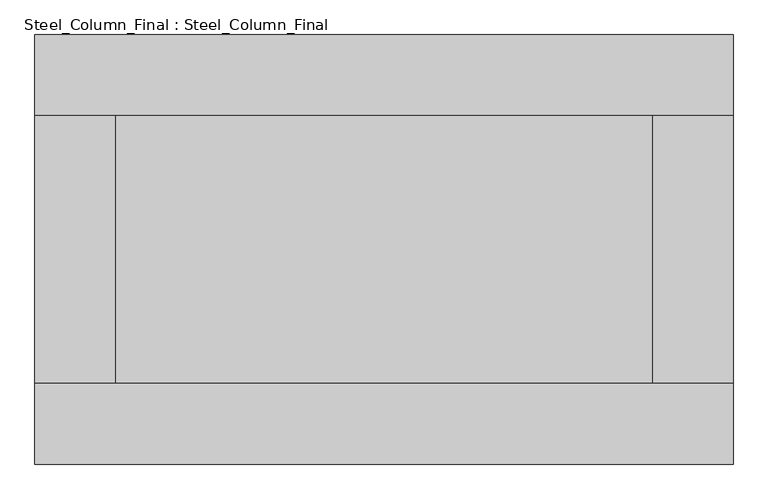
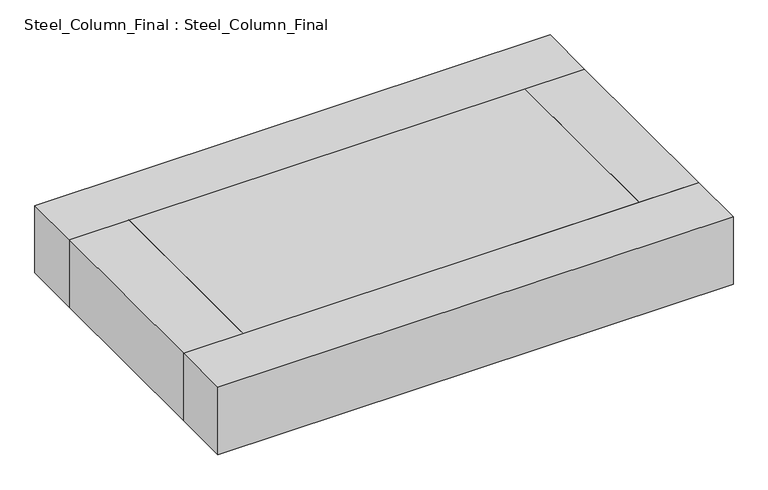
"""IFC4 building model written with IfcOpenShell, lengths in millimetres: proxy geometry, Steel_Column_Final : Steel_Column_Final."""

from ifc_helpers import new_model, si_unit, frame, origin, place, context, project, spatial, polyline, outline, extrude, source, transform, mapped, element, save


def steel_column_final_steel_column_final_b25c4c34(model_context):
    return source(origin(), model_context, "Body", "SweptSolid", [
        extrude(outline(polyline([(6500.0, 2500.0), (-6500.0, 2500.0), (-6500.0, 4000.0), (6500.0, 4000.0), (6500.0, 2500.0)])), frame((0.0, 0.0, 46130.0), z_axis=(0.0, 0.0, 1.0), x_axis=(1.0, 0.0, 0.0)), (0.0, 0.0, 1.0), 1800.0),
        extrude(outline(polyline([(-6500.0, -2500.0), (6500.0, -2500.0), (6500.0, -4000.0), (-6500.0, -4000.0), (-6500.0, -2500.0)])), frame((0.0, 0.0, 46130.0), z_axis=(0.0, 0.0, 1.0), x_axis=(1.0, 0.0, 0.0)), (0.0, 0.0, 1.0), 1800.0),
        extrude(outline(polyline([(5000.0, -2500.0), (5000.0, 2500.0), (6500.0, 2500.0), (6500.0, -2500.0), (5000.0, -2500.0)])), frame((0.0, 0.0, 46130.0), z_axis=(0.0, 0.0, 1.0), x_axis=(1.0, 0.0, 0.0)), (0.0, 0.0, 1.0), 1800.0),
        extrude(outline(polyline([(-5000.0, 2500.0), (-5000.0, -2500.0), (-6500.0, -2500.0), (-6500.0, 2500.0), (-5000.0, 2500.0)])), frame((0.0, 0.0, 46130.0), z_axis=(0.0, 0.0, 1.0), x_axis=(1.0, 0.0, 0.0)), (0.0, 0.0, 1.0), 1800.0),
        extrude(outline(polyline([(-5000.0, -2500.0), (-5000.0, 2500.0), (5000.0, 2500.0), (5000.0, -2500.0), (-5000.0, -2500.0)])), frame((0.0, 0.0, 46130.0), z_axis=(0.0, 0.0, 1.0), x_axis=(1.0, 0.0, 0.0)), (0.0, 0.0, 1.0), 1800.0),
    ])


if __name__ == "__main__":
    model = new_model("IFC4")
    model_context = context("Model", 3, world=origin())
    ifc_project = project(units=[si_unit("LENGTHUNIT", "METRE", prefix="MILLI")], contexts=[model_context])
    site = spatial("IfcSite", under=ifc_project)
    building = spatial("IfcBuilding", under=site)
    placement = place(None, origin())
    steel_column_final_steel_column_final_shape = steel_column_final_steel_column_final_b25c4c34(model_context)
    element("IfcBuildingElementProxy", 1, Name="Steel_Column_Final : Steel_Column_Final", ObjectType="Steel_Column_Final : Steel_Column_Final", at=placement, inside=building, context=model_context, shape_type="MappedRepresentation", body=[
        mapped(steel_column_final_steel_column_final_shape, transform((0.0, 0.0, 0.0), x_axis=(1.0, 0.0, 0.0), y_axis=(0.0, 1.0, 0.0), z_axis=(0.0, 0.0, 1.0))),
    ])
    save(model, "model.ifc")

# Revit data of these elements
# Type "Steel_Column_Final : Steel_Column_Final"
#   Top Width [instance default] = 5000 mm
#   Top Length = 10000 mm
#   Length = 21000 mm
#   Height [instance default] = 50000 mm
#   Bottom Width [instance default] = 5000 mm
#   Default Elevation = 0
# Element 1 (IfcBuildingElementProxy, "Steel_Column_Final : Steel_Column_Final")
#   Height = 46130 mm
